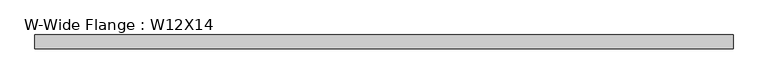
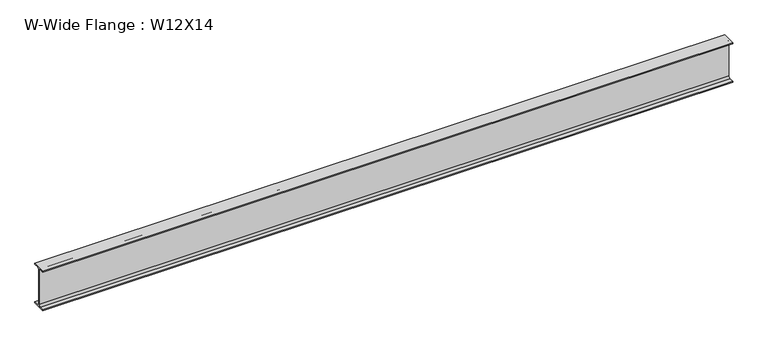
"""IFC4 building model written with IfcOpenShell, lengths in millimetres: beam geometry, W-Wide Flange : W12X14."""

from ifc_helpers import new_model, si_unit, point, frame, frame_2d, origin, place, context, project, spatial, polyline, circle_curve, trimmed, segment, composite_curve, outline, extrude, source, transform, mapped, element, save


def w_wide_flange_w12x14_e5c78693(model_context):
    return source(origin(), model_context, "Body", "SweptSolid", [
        extrude(outline(composite_curve([segment(polyline([(50.419, -145.415), (50.419, -151.13), (-50.419, -151.13), (-50.419, -145.415), (-15.875, -145.415)]), True, "CONTINUOUS"), segment(trimmed(circle_curve(frame_2d((-15.875, -132.08)), 13.335), [point((-15.875, -145.415))], [point((-2.54, -132.08))], True, "CARTESIAN"), True, "CONTINUOUS"), segment(polyline([(-2.54, -132.08), (-2.54, 132.08)]), True, "CONTINUOUS"), segment(trimmed(circle_curve(frame_2d((-15.875, 132.08)), 13.335), [point((-2.54, 132.08))], [point((-15.875, 145.415))], True, "CARTESIAN"), True, "CONTINUOUS"), segment(polyline([(-15.875, 145.415), (-50.419, 145.415), (-50.419, 151.13), (50.419, 151.13), (50.419, 145.415), (15.875, 145.415)]), True, "CONTINUOUS"), segment(trimmed(circle_curve(frame_2d((15.875, 132.08)), 13.335), [point((15.875, 145.415))], [point((2.54, 132.08))], True, "CARTESIAN"), True, "CONTINUOUS"), segment(polyline([(2.54, 132.08), (2.54, -132.08)]), True, "CONTINUOUS"), segment(trimmed(circle_curve(frame_2d((15.875, -132.08)), 13.335), [point((2.54, -132.08))], [point((15.875, -145.415))], True, "CARTESIAN"), True, "CONTINUOUS"), segment(polyline([(15.875, -145.415), (50.419, -145.415)]), True, "CONTINUOUS")], self_intersect=False)), frame((-2514.092, 0.0, 0.0), z_axis=(1.0, 0.0, 0.0), x_axis=(0.0, 1.0, 0.0)), (0.0, 0.0, 1.0), 5028.184),
    ])


if __name__ == "__main__":
    model = new_model("IFC4")
    model_context = context("Model", 3, world=origin())
    ifc_project = project(units=[si_unit("LENGTHUNIT", "METRE", prefix="MILLI")], contexts=[model_context])
    site = spatial("IfcSite", under=ifc_project)
    building = spatial("IfcBuilding", under=site)
    placement = place(None, origin())
    w_wide_flange_w12x14_shape = w_wide_flange_w12x14_e5c78693(model_context)
    element("IfcBeam", 1, ObjectType="W-Wide Flange : W12X14", at=placement, inside=building, context=model_context, shape_type="MappedRepresentation", body=[
        mapped(w_wide_flange_w12x14_shape, transform((0.0, 0.0, 0.0), x_axis=(1.0, 0.0, 0.0), y_axis=(0.0, 1.0, 0.0), z_axis=(0.0, 0.0, 1.0))),
    ])
    save(model, "model.ifc")

# Revit data of these elements
# Type "W-Wide Flange : W12X14"
#   Assembly Code = "B10"
#   W = 14
#   Length [instance default] = 5' - 0"
#   bf = 0' - 3.97"
#   d = 0' - 11.9"
#   k = 0' - 0 3/4"
#   k2 = 0' - 0.525"
#   tf = 0' - 0.225"
#   tw = 0' - 0.2"
#   A = 0.0288889 SF
#   Structural Material [instance default] = Steel ASTM A992
# Element 1 (IfcBeam, "W-Wide Flange : W12X14")
#   Materials on its faces: "Steel ASTM A992"
# Materials
#   "Steel ASTM A992": class "Metal", colour RGB 199 199 199, transparency 0, Description = "Structural steel 50ksi", Cost = 0
